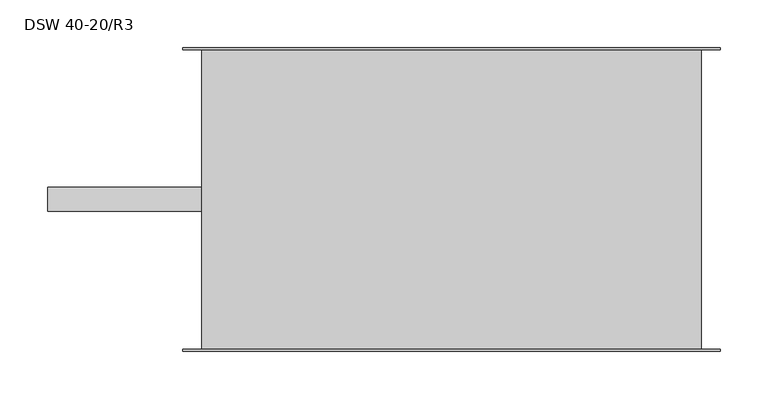
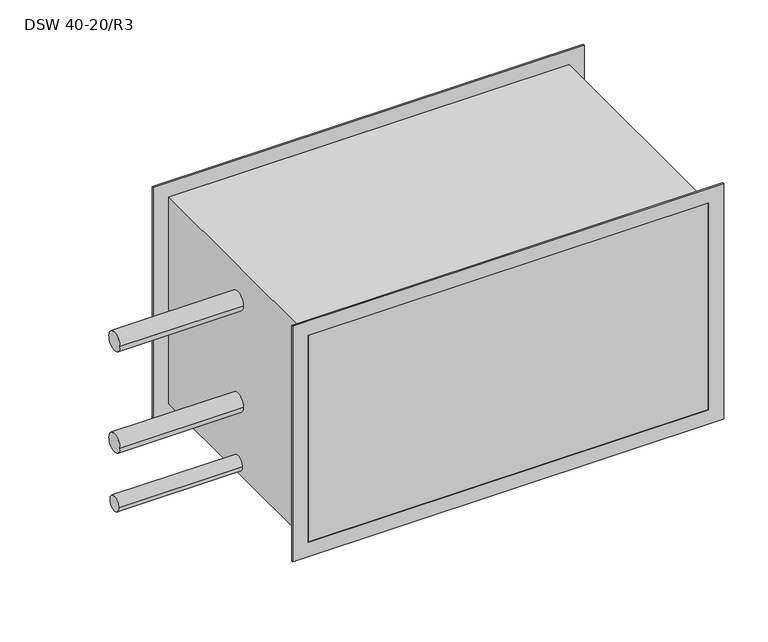
"""IFC4 building model written with IfcOpenShell, lengths in millimetres: proxy geometry, Воздухоохладитель водяной DSW : DSW 40-20/R3."""

from ifc_helpers import new_model, si_unit, point, frame, frame_2d, origin, place, context, project, spatial, polyline, circle_curve, trimmed, segment, composite_curve, outline, extrude, source, transform, mapped, element, save


def dsw_40_20_r3_bd0e4b4a(model_context):
    return source(origin(), model_context, "Body", "SweptSolid", [
        extrude(outline(composite_curve([segment(trimmed(circle_curve(frame_2d((0.0, 95.0)), 12.5), [point((-12.5, 95.0))], [point((12.5, 95.0))], False, "CARTESIAN"), True, "CONTINUOUS"), segment(trimmed(circle_curve(frame_2d((0.0, 95.0)), 12.5), [point((12.5, 95.0))], [point((-12.5, 95.0))], False, "CARTESIAN"), True, "CONTINUOUS")], self_intersect=False)), frame((-422.0, 0.0, 0.0), z_axis=(1.0, 0.0, 0.0), x_axis=(0.0, 1.0, 0.0)), (0.0, 0.0, 1.0), 161.0),
        extrude(outline(composite_curve([segment(trimmed(circle_curve(frame_2d((0.0, -129.0)), 10.0), [point((-10.0, -129.0))], [point((10.0, -129.0))], False, "CARTESIAN"), True, "CONTINUOUS"), segment(trimmed(circle_curve(frame_2d((0.0, -129.0)), 10.0), [point((10.0, -129.0))], [point((-10.0, -129.0))], False, "CARTESIAN"), True, "CONTINUOUS")], self_intersect=False)), frame((-422.0, 0.0, 0.0), z_axis=(1.0, 0.0, 0.0), x_axis=(0.0, 1.0, 0.0)), (0.0, 0.0, 1.0), 161.0),
        extrude(outline(composite_curve([segment(trimmed(circle_curve(frame_2d((0.0, -45.0)), 12.5), [point((-12.5, -45.0))], [point((12.5, -45.0))], False, "CARTESIAN"), True, "CONTINUOUS"), segment(trimmed(circle_curve(frame_2d((0.0, -45.0)), 12.5), [point((12.5, -45.0))], [point((-12.5, -45.0))], False, "CARTESIAN"), True, "CONTINUOUS")], self_intersect=False)), frame((-422.0, 0.0, 0.0), z_axis=(1.0, 0.0, 0.0), x_axis=(0.0, 1.0, 0.0)), (0.0, 0.0, 1.0), 161.0),
        extrude(outline(polyline([(162.5, 281.0), (162.5, -281.0), (-162.5, -281.0), (-162.5, 281.0), (162.5, 281.0)]), holes=[polyline([(-142.5, 261.0), (-142.5, -261.0), (142.5, -261.0), (142.5, 261.0), (-142.5, 261.0)])]), frame((0.0, 156.5, 0.0), z_axis=(0.0, 1.0, 0.0), x_axis=(0.0, 0.0, 1.0)), (0.0, 0.0, 1.0), 2.0),
        extrude(outline(polyline([(162.5, -281.0), (-162.5, -281.0), (-162.5, 281.0), (162.5, 281.0), (162.5, -281.0)]), holes=[polyline([(142.5, 261.0), (-142.5, 261.0), (-142.5, -261.0), (142.5, -261.0), (142.5, 261.0)])]), frame((0.0, -158.5, 0.0), z_axis=(0.0, 1.0, 0.0), x_axis=(0.0, 0.0, 1.0)), (0.0, 0.0, 1.0), 2.0),
        extrude(outline(polyline([(261.0, -158.5), (-261.0, -158.5), (-261.0, 158.5), (261.0, 158.5), (261.0, -158.5)])), frame((0.0, 0.0, -142.5), z_axis=(0.0, 0.0, 1.0), x_axis=(1.0, 0.0, 0.0)), (0.0, 0.0, 1.0), 285.0),
    ])


if __name__ == "__main__":
    model = new_model("IFC4")
    model_context = context("Model", 3, world=origin())
    ifc_project = project(units=[si_unit("LENGTHUNIT", "METRE", prefix="MILLI")], contexts=[model_context])
    site = spatial("IfcSite", under=ifc_project)
    building = spatial("IfcBuilding", under=site)
    placement = place(None, origin())
    dsw_40_20_r3_shape = dsw_40_20_r3_bd0e4b4a(model_context)
    element("IfcBuildingElementProxy", 1, Name="Воздухоохладитель водяной DSW : DSW 40-20/R3", ObjectType="Воздухоохладитель водяной DSW : DSW 40-20/R3", at=placement, inside=building, context=model_context, shape_type="MappedRepresentation", body=[
        mapped(dsw_40_20_r3_shape, transform((0.0, 0.0, 0.0), x_axis=(1.0, 0.0, 0.0), y_axis=(0.0, 1.0, 0.0), z_axis=(0.0, 0.0, 1.0))),
    ])
    save(model, "model.ifc")

# Revit data of these elements
# Type "Воздухоохладитель водяной DSW : DSW 40-20/R3"
#   Manufacturer = "WAER"
#   URL = "https://waer-air.com/"
#   ADSK_Система_Имя [instance default] = ""
#   ADSK_Наименование краткое = "DSW 40-20/R3"
#   ADSK_Наименование = "Воздухоохладитель водяной DSW 40-20/R3"
#   ADSK_Масса_Текст = "16.5"
#   ADSK_Марка = ""
#   ADSK_Код изделия = ""
#   ADSK_Завод-изготовитель = "WAER"
#   ADSK_Единица измерения = "шт."
#   Д = 622 mm
#   Б = 285 mm
#   А = 522 mm
#   ADSK_Расход воздуха = 0 m³/h
#   ADSK_Размер_Ширина = 400 mm
#   ADSK_Размер_Диаметр дренаж = 20 mm
#   ADSK_Размер_Диаметр ТО = 25 mm
#   ADSK_Размер_Высота = 200 mm
#   ADSK_Потеря давления воздуха = 0.0 Pa
#   ADSK_Масса = 16.5
#   ADSK_Количество = 1
#   Default Elevation = 0
#   Keynote = ""
